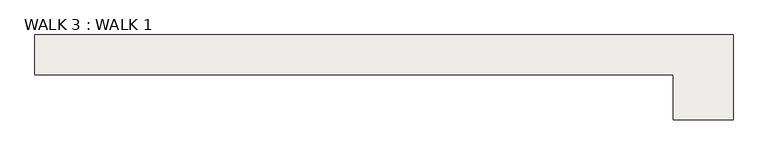
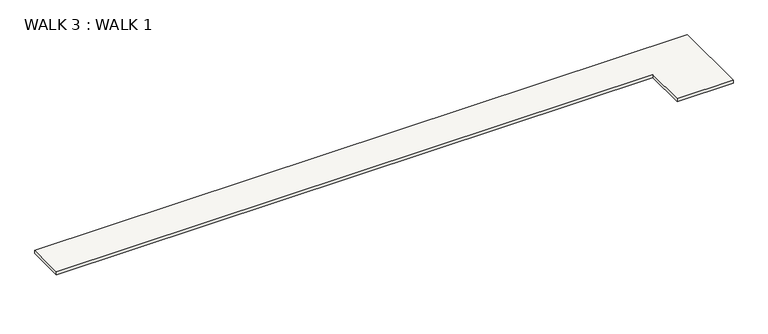
"""IFC4 building model written with IfcOpenShell, lengths in millimetres: slab geometry, WALK 3 : WALK 1."""

import ifcopenshell
import ifcopenshell.guid

model = None  # the IFC model being written
_history = None  # IfcOwnerHistory: only IFC2X3 demands one
_inside = {}  # id of a spatial element -> (the spatial element, [elements in it])
_under = {}  # id of a project, library or spatial element -> (it, [spatial elements below it])
_declared = {}  # id of a project -> (the project, [libraries it declares])
_typed = {}  # id of a type object -> (the type object, [elements of that type])
_made_of = {}  # id of a material, layer set ... -> (it, [elements and type objects made of it])


def new_model(schema):
    """Start an empty IFC model of exactly this schema.

    Asked for "IFC4X3", IfcOpenShell would pick the latest addendum, in which some entities
    have other attributes; the version numbers below select the first issue.
    IFC2X3 requires an IfcOwnerHistory on every rooted entity: one is made here for all.
    """
    global model, _history
    if schema == "IFC4X3":
        model = ifcopenshell.file(schema_version=(4, 3, 0, 0))
    else:
        model = ifcopenshell.file(schema=schema)
    _inside.clear()
    _under.clear()
    _declared.clear()
    _typed.clear()
    _made_of.clear()
    _history = None
    if model.schema == "IFC2X3":
        org = make("IfcOrganization", Name="unknown")
        user = make(
            "IfcPersonAndOrganization",
            ThePerson=make("IfcPerson", FamilyName="unknown"),
            TheOrganization=org,
        )
        app = make(
            "IfcApplication",
            ApplicationDeveloper=org,
            Version="unknown",
            ApplicationFullName="unknown",
            ApplicationIdentifier="unknown",
        )
        _history = make(
            "IfcOwnerHistory",
            OwningUser=user,
            OwningApplication=app,
            ChangeAction="ADDED",
            CreationDate=0,
        )
    return model


def make(cls, **values):
    """One entity of the class cls with the attributes given. An attribute that is None is left unset."""
    return model.create_entity(
        cls, **{name: value for name, value in values.items() if value is not None}
    )


def rooted(cls, **values):
    """An entity with a GlobalId (a new one), such as an element, a storey or a relation."""
    return make(cls, GlobalId=ifcopenshell.guid.new(), OwnerHistory=_history, **values)


def si_unit(unit_type, name, prefix=None):
    """IfcSIUnit, for example si_unit("LENGTHUNIT", "METRE", prefix="MILLI")."""
    return make("IfcSIUnit", UnitType=unit_type, Prefix=prefix, Name=name)


def assignment(units):
    """IfcUnitAssignment: the units of a project."""
    return None if units is None else make("IfcUnitAssignment", Units=units)


def point(xyz):
    """IfcCartesianPoint."""
    return None if xyz is None else make("IfcCartesianPoint", Coordinates=xyz)


def direction(xyz):
    """IfcDirection."""
    return None if xyz is None else make("IfcDirection", DirectionRatios=xyz)


def frame(location, z_axis=None, x_axis=None):
    """IfcAxis2Placement3D, a coordinate frame: its origin and axes. An axis left out is left unset."""
    return make(
        "IfcAxis2Placement3D",
        Location=point(location),
        Axis=direction(z_axis),
        RefDirection=direction(x_axis),
    )


def origin():
    """The frame at (0, 0, 0) with its axes left unset."""
    return frame((0.0, 0.0, 0.0))


def place(relative_to, where):
    """IfcLocalPlacement: puts the frame where relative to a parent placement (None: the world)."""
    return make(
        "IfcLocalPlacement", PlacementRelTo=relative_to, RelativePlacement=where
    )


def context(
    kind, dimensions, precision=None, world=None, true_north=None, identifier=None
):
    """IfcGeometricRepresentationContext, for example the 3D "Model" context."""
    return make(
        "IfcGeometricRepresentationContext",
        ContextIdentifier=identifier,
        ContextType=kind,
        CoordinateSpaceDimension=dimensions,
        Precision=precision,
        WorldCoordinateSystem=world,
        TrueNorth=true_north,
    )


def project(units=None, contexts=None):
    """IfcProject with its units and contexts."""
    return rooted(
        "IfcProject",
        Name="project",
        RepresentationContexts=contexts,
        UnitsInContext=assignment(units),
    )


def spatial(cls, under=None, at=None, **own):
    """A site, building, storey or space (cls), placed at a placement, below another one or the project."""
    s = rooted(cls, ObjectPlacement=at, **own)
    if under is not None:
        _under.setdefault(under.id(), (under, []))[1].append(s)
    return s


def polyline(points):
    """IfcPolyline through the points."""
    return make("IfcPolyline", Points=[point(p) for p in points])


def outline(outer, holes=None, kind="AREA"):
    """IfcArbitraryClosedProfileDef: a profile drawn as a closed curve; with holes, ...WithVoids."""
    if holes is None:
        return make("IfcArbitraryClosedProfileDef", ProfileType=kind, OuterCurve=outer)
    return make(
        "IfcArbitraryProfileDefWithVoids",
        ProfileType=kind,
        OuterCurve=outer,
        InnerCurves=holes,
    )


def extrude(swept, where, along, depth):
    """IfcExtrudedAreaSolid: the profile swept, set in the frame where, extruded along a direction by depth."""
    return make(
        "IfcExtrudedAreaSolid",
        SweptArea=swept,
        Position=where,
        ExtrudedDirection=direction(along),
        Depth=depth,
    )


def shape(context_of_items, identifier, shape_type, items):
    """IfcShapeRepresentation: the items that make up one representation, for example the "Body"."""
    return make(
        "IfcShapeRepresentation",
        ContextOfItems=context_of_items,
        RepresentationIdentifier=identifier,
        RepresentationType=shape_type,
        Items=items,
    )


def source(mapping_origin, context_of_items, identifier, shape_type, items):
    """IfcRepresentationMap: a shape defined once, which mapped items show again and again."""
    return make(
        "IfcRepresentationMap",
        MappingOrigin=mapping_origin,
        MappedRepresentation=shape(context_of_items, identifier, shape_type, items),
    )


def transform(
    local_origin,
    x_axis=None,
    y_axis=None,
    z_axis=None,
    scale=None,
    scale2=None,
    scale3=None,
    uniform=True,
):
    """IfcCartesianTransformationOperator3D, or its non-uniform kind. x_axis, y_axis, z_axis: its Axis1, 2, 3."""
    if uniform:
        return make(
            "IfcCartesianTransformationOperator3D",
            Axis1=direction(x_axis),
            Axis2=direction(y_axis),
            LocalOrigin=point(local_origin),
            Scale=scale,
            Axis3=direction(z_axis),
        )
    return make(
        "IfcCartesianTransformationOperator3DnonUniform",
        Axis1=direction(x_axis),
        Axis2=direction(y_axis),
        LocalOrigin=point(local_origin),
        Scale=scale,
        Axis3=direction(z_axis),
        Scale2=scale2,
        Scale3=scale3,
    )


def mapped(mapping_source, mapping_target):
    """IfcMappedItem: shows the shape of a source again, moved by a transform."""
    return make(
        "IfcMappedItem", MappingSource=mapping_source, MappingTarget=mapping_target
    )


def made_of(thing, what):
    """Note that an element or type object is made of a material, layer set ...; save() writes the relation."""
    if what is not None:
        _made_of.setdefault(what.id(), (what, []))[1].append(thing)
    return thing


def element(
    cls,
    number,
    at=None,
    inside=None,
    cuts=None,
    type_object=None,
    material=None,
    context=None,
    identifier="Body",
    shape_type=None,
    held_by="IfcProductDefinitionShape",
    body=None,
    shapes=None,
    **own,
):
    """One element of the class cls, such as IfcWall. Its Tag is "e" and its number.

    at: its placement. inside: the storey or other place that contains it. cuts: it is an
    opening in that element (IfcRelVoidsElement). A single representation is given by context,
    identifier, shape_type and body (its items); several are given by shapes. held_by: the class
    of the entity that holds the representations. save() writes the other relations.
    """
    e = rooted(cls, Tag="e%d" % number, ObjectPlacement=at, **own)
    if body is not None:
        shapes = [shape(context, identifier, shape_type, body)]
    if shapes is not None:
        e.Representation = make(held_by, Representations=shapes)
    if inside is not None:
        _inside.setdefault(inside.id(), (inside, []))[1].append(e)
    if cuts is not None:
        rooted(
            "IfcRelVoidsElement", RelatingBuildingElement=cuts, RelatedOpeningElement=e
        )
    if type_object is not None:
        _typed.setdefault(type_object.id(), (type_object, []))[1].append(e)
    return made_of(e, material)


def aggregate(whole, parts):
    """IfcRelAggregates: a whole, such as a stair, and the parts it consists of."""
    return rooted("IfcRelAggregates", RelatingObject=whole, RelatedObjects=parts)


def save(model, path):
    """Write the relations noted so far, then the file.

    IfcRelAggregates (storeys below a building ...), IfcRelContainedInSpatialStructure (elements
    in a storey), IfcRelDefinesByType, IfcRelAssociatesMaterial and IfcRelDeclares: one each for
    every whole, place, type object, material and project.
    """
    for whole, parts in _under.values():
        aggregate(whole, parts)
    for where, things in _inside.values():
        rooted(
            "IfcRelContainedInSpatialStructure",
            RelatedElements=things,
            RelatingStructure=where,
        )
    for kind, things in _typed.values():
        rooted("IfcRelDefinesByType", RelatedObjects=things, RelatingType=kind)
    for what, things in _made_of.values():
        rooted("IfcRelAssociatesMaterial", RelatedObjects=things, RelatingMaterial=what)
    for by, libraries in _declared.values():
        rooted("IfcRelDeclares", RelatingContext=by, RelatedDefinitions=libraries)
    model.write(path)


def walk_3_walk_1_14dd6b5e(model_context):
    return source(origin(), model_context, "Body", "SweptSolid", [
        extrude(outline(polyline([(341.9325037, -23029.3506192), (-9411.6674963, -23029.3506192), (-9411.6674963, -22419.7506192), (1256.3325037, -22419.7506192), (1256.3325037, -23715.1506192), (341.9325037, -23715.1506192), (341.9325037, -23029.3506192)])), frame((0.0, 0.0, 3810.0), z_axis=(0.0, 0.0, 1.0), x_axis=(1.0, 0.0, 0.0)), (0.0, 0.0, 1.0), 50.8),
    ])


if __name__ == "__main__":
    model = new_model("IFC4")
    model_context = context("Model", 3, world=origin())
    ifc_project = project(units=[si_unit("LENGTHUNIT", "METRE", prefix="MILLI")], contexts=[model_context])
    site = spatial("IfcSite", under=ifc_project)
    building = spatial("IfcBuilding", under=site)
    placement = place(None, origin())
    walk_3_walk_1_shape = walk_3_walk_1_14dd6b5e(model_context)
    element("IfcSlab", 1, ObjectType="WALK 3 : WALK 1", at=placement, inside=building, context=model_context, shape_type="MappedRepresentation", body=[
        mapped(walk_3_walk_1_shape, transform((0.0, 0.0, 0.0), x_axis=(1.0, 0.0, 0.0), y_axis=(0.0, 1.0, 0.0), z_axis=(0.0, 0.0, 1.0))),
    ])
    save(model, "model.ifc")

# Revit data of these elements
# Element 1 (IfcSlab, "WALK 3 : WALK 1")
#   Materials on its faces: "Default Floor"
# Materials
#   "Default Floor": class "Miscellaneous", colour RGB 128 128 128, transparency 0
